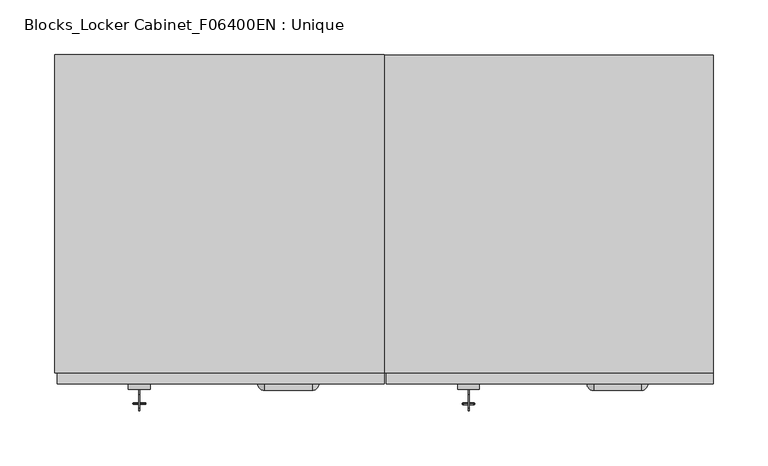
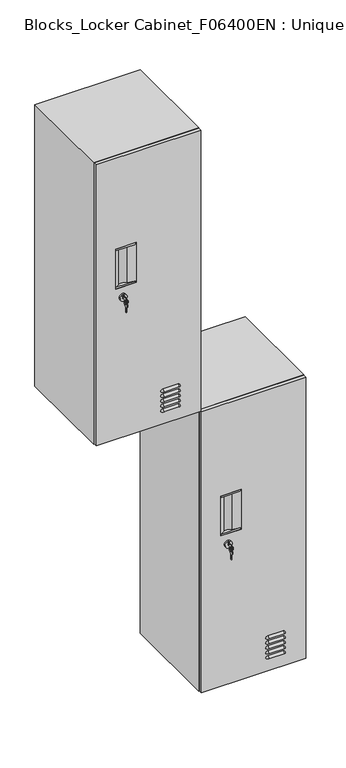
"""IFC4 building model written with IfcOpenShell, lengths in millimetres: furniture geometry, Blocks_Locker Cabinet_F06400EN : Unique."""

from ifc_helpers import new_model, si_unit, point, frame, frame_2d, origin, place, context, project, spatial, polyline, circle_curve, ellipse_curve, trimmed, segment, composite_curve, outline, extrude, faceted_brep, source, transform, mapped, element, save
from ifc_brep_helpers import plane_surface, cylinder_surface, revolved_surface, advanced_brep


def blocks_locker_cabinet_f06400en_unique_78fff643(model_context):
    return source(origin(), model_context, "Body", "SolidModel", [
        advanced_brep(
        [(-383.0, -12.5, 1375.0), (-363.0, -12.5, 1375.0), (-371.1588195, -12.5, 1382.0962926), (-371.1588195, -12.5, 1372.8618188), (-374.8411805, -12.5, 1372.8618188), (-374.8411805, -12.5, 1382.0962926), (-383.0, -7.5, 1375.0), (-363.0, -7.5, 1375.0), (-383.0, -10.7450625, 1375.0), (-363.0, -10.7450625, 1375.0), (-371.1588195, -10.7450625, 1382.0962926), (-371.1588195, -10.7450625, 1372.8618188), (-374.8411805, -10.7450625, 1372.8618188), (-374.8411805, -10.7450625, 1382.0962926)],
        [
            (0, 1, circle_curve(frame((-373.0, -12.5, 1375.0), z_axis=(0.0, -1.0, 0.0), x_axis=(1.0, 0.0, 0.0)), 10.0)),
            (1, 0, circle_curve(frame((-373.0, -12.5, 1375.0), z_axis=(0.0, -1.0, 0.0), x_axis=(1.0, 0.0, 0.0)), 10.0)),
            (2, 3),
            (3, 4),
            (4, 5),
            (5, 2),
            (6, 7, circle_curve(frame((-373.0, -7.5, 1375.0), z_axis=(0.0, 1.0, 0.0), x_axis=(1.0, 0.0, 0.0)), 10.0)),
            (7, 6, circle_curve(frame((-373.0, -7.5, 1375.0), z_axis=(0.0, 1.0, 0.0), x_axis=(1.0, 0.0, 0.0)), 10.0)),
            (0, 8),
            (8, 6),
            (7, 9),
            (9, 1),
            (2, 10),
            (10, 11),
            (11, 3),
            (11, 12),
            (12, 4),
            (12, 13),
            (13, 5),
            (13, 10),
        ],
        [
            plane_surface(frame((-363.0, -12.5, 1375.0), z_axis=(0.0, -1.0, 0.0), x_axis=(0.0, 0.0, 1.0))),
            plane_surface(frame((-363.0, -7.5, 1375.0), z_axis=(0.0, 1.0, 0.0), x_axis=(0.0, 0.0, -1.0))),
            cylinder_surface(frame((-373.0, -7.5, 1375.0), z_axis=(0.0, -1.0, 0.0), x_axis=(1.0, 0.0, 0.0)), 10.0),
            plane_surface(frame((-371.1588195, -12.5, 1382.0962926), z_axis=(-1.0, 0.0, 0.0), x_axis=(0.0, 1.0, 0.0))),
            plane_surface(frame((-371.1588195, -12.5, 1372.8618188), z_axis=(0.0, 0.0, 1.0), x_axis=(0.0, 1.0, 0.0))),
            plane_surface(frame((-374.8411805, -12.5, 1372.8618188), z_axis=(1.0, 0.0, 0.0), x_axis=(0.0, 1.0, 0.0))),
            plane_surface(frame((-374.8411805, -12.5, 1382.0962926), z_axis=(0.0, 0.0, -1.0), x_axis=(0.0, 1.0, 0.0))),
            plane_surface(frame((-363.0, -10.7450625, 1375.0), z_axis=(0.0, -1.0, 0.0), x_axis=(0.0, 0.0, 1.0))),
        ],
        [
            (0, [[1, 2], [3, 4, 5, 6]]),
            (1, [[7, 8]]),
            (2, [[-1, 9, 10, -8, 11, 12]]),
            (2, [[-2, -12, -11, -7, -10, -9]]),
            (3, [[-3, 13, 14, 15]]),
            (4, [[-4, -15, 16, 17]]),
            (5, [[-5, -17, 18, 19]]),
            (6, [[-6, -19, 20, -13]]),
            (7, [[-14, -20, -18, -16]]),
        ],
    ),
        extrude(outline(composite_curve([segment(trimmed(circle_curve(frame_2d((-23.0067332, 1375.0)), 6.5414185), [point((-16.8246351, 1372.8618188))], [point((-17.0336838, 1377.6669902))], False, "CARTESIAN"), True, "CONTINUOUS"), segment(polyline([(-17.0336838, 1377.6669902), (-10.7450625, 1377.6669902), (-10.7450625, 1372.8618188), (-12.0321832, 1372.8618188)]), True, "CONTINUOUS"), segment(trimmed(circle_curve(frame_2d((-12.908516, 1372.8618188)), 0.8763328), [point((-12.0321832, 1372.8618188))], [point((-13.7848488, 1372.8618188))], True, "CARTESIAN"), True, "CONTINUOUS"), segment(polyline([(-13.7848488, 1372.8618188), (-16.8246351, 1372.8618188)]), True, "CONTINUOUS")], self_intersect=False), holes=[composite_curve([segment(trimmed(circle_curve(frame_2d((-25.6281997, 1375.0)), 1.688217), [point((-27.3164167, 1375.0))], [point((-23.9399827, 1375.0))], True, "CARTESIAN"), True, "CONTINUOUS"), segment(trimmed(circle_curve(frame_2d((-25.6281997, 1375.0)), 1.688217), [point((-23.9399827, 1375.0))], [point((-27.3164167, 1375.0))], True, "CARTESIAN"), True, "CONTINUOUS")], self_intersect=False)]), frame((-373.4043078, 0.0, 0.0), z_axis=(1.0, 0.0, 0.0), x_axis=(0.0, 1.0, 0.0)), (0.0, 0.0, 1.0), 0.9157402),
        extrude(outline(composite_curve([segment(trimmed(circle_curve(frame_2d((-25.6743188, 1360.9839856)), 6.5414185), [point((-27.8125, 1354.8018875))], [point((-24.2573286, 1354.5978839))], False, "CARTESIAN"), True, "CONTINUOUS"), segment(polyline([(-24.2573286, 1354.5978839), (-24.2573286, 1337.7095301), (-25.9613419, 1337.7095301), (-27.8125, 1340.3532579), (-27.8125, 1342.0094356)]), True, "CONTINUOUS"), segment(trimmed(circle_curve(frame_2d((-27.8125, 1342.8857684)), 0.8763328), [point((-27.8125, 1342.0094356))], [point((-27.8125, 1343.7621012))], True, "CARTESIAN"), True, "CONTINUOUS"), segment(polyline([(-27.8125, 1343.7621012), (-27.8125, 1346.0094356)]), True, "CONTINUOUS"), segment(trimmed(circle_curve(frame_2d((-27.8125, 1346.8857684)), 0.8763328), [point((-27.8125, 1346.0094356))], [point((-27.8125, 1347.7621012))], True, "CARTESIAN"), True, "CONTINUOUS"), segment(polyline([(-27.8125, 1347.7621012), (-27.8125, 1350.0094356)]), True, "CONTINUOUS"), segment(trimmed(circle_curve(frame_2d((-27.8125, 1350.8857684)), 0.8763328), [point((-27.8125, 1350.0094356))], [point((-27.8125, 1351.7621012))], True, "CARTESIAN"), True, "CONTINUOUS"), segment(polyline([(-27.8125, 1351.7621012), (-27.8125, 1354.8018875)]), True, "CONTINUOUS")], self_intersect=False), holes=[composite_curve([segment(trimmed(circle_curve(frame_2d((-25.6743188, 1363.6054521)), 1.688217), [point((-25.6743188, 1365.2936691))], [point((-25.6743188, 1361.9172351))], True, "CARTESIAN"), True, "CONTINUOUS"), segment(trimmed(circle_curve(frame_2d((-25.6743188, 1363.6054521)), 1.688217), [point((-25.6743188, 1361.9172351))], [point((-25.6743188, 1365.2936691))], True, "CARTESIAN"), True, "CONTINUOUS")], self_intersect=False)]), frame((-373.4043078, 0.0, 0.0), z_axis=(1.0, 0.0, 0.0), x_axis=(0.0, 1.0, 0.0)), (0.0, 0.0, 1.0), 0.9157402),
        advanced_brep(
        [(-368.8, -25.663019, 1369.4000012), (-377.2, -25.663019, 1369.4000012), (-378.8, -25.663019, 1369.4000012), (-367.2, -25.663019, 1369.4000012)],
        [
            (0, 1, circle_curve(frame((-373.0, -25.663019, 1369.4000012), z_axis=(0.0, 1.0, 0.0), x_axis=(-1.0, 0.0, 0.0)), 4.2)),
            (1, 2, circle_curve(frame((-378.0, -25.663019, 1369.4000012), z_axis=(0.0, 0.0, -1.0), x_axis=(1.0, 0.0, 0.0)), 0.8)),
            (2, 3, circle_curve(frame((-373.0, -25.663019, 1369.4000012), z_axis=(0.0, -1.0, 0.0), x_axis=(-1.0, 0.0, 0.0)), 5.8)),
            (3, 0, circle_curve(frame((-368.0, -25.663019, 1369.4000012), z_axis=(0.0, 0.0, -1.0), x_axis=(-1.0, 0.0, 0.0)), 0.8)),
            (2, 1, circle_curve(frame((-378.0, -25.663019, 1369.4000012), z_axis=(0.0, 0.0, -1.0), x_axis=(1.0, 0.0, 0.0)), 0.8)),
            (0, 3, circle_curve(frame((-368.0, -25.663019, 1369.4000012), z_axis=(0.0, 0.0, -1.0), x_axis=(-1.0, 0.0, 0.0)), 0.8)),
            (1, 0, circle_curve(frame((-373.0, -25.663019, 1369.4000012), z_axis=(0.0, 1.0, 0.0), x_axis=(1.0, 0.0, 0.0)), 4.2)),
            (3, 2, circle_curve(frame((-373.0, -25.663019, 1369.4000012), z_axis=(0.0, -1.0, 0.0), x_axis=(1.0, 0.0, 0.0)), 5.8)),
        ],
        [
            revolved_surface(trimmed(ellipse_curve(frame((-378.0, -25.663019, 1369.4000012), z_axis=(0.0, 0.0, 1.0), x_axis=(1.0, 0.0, 0.0)), 0.8, 0.8), [point((-378.8, -25.663019, 1369.4000012))], [point((-377.2, -25.663019, 1369.4000012))], True, "CARTESIAN"), (-373.0, 2.5, 1369.4000012), (0.0, -1.0, 0.0)),
            revolved_surface(trimmed(ellipse_curve(frame((-378.0, -25.663019, 1369.4000012), z_axis=(0.0, 0.0, 1.0), x_axis=(1.0, 0.0, 0.0)), 0.8, 0.8), [point((-377.2, -25.663019, 1369.4000012))], [point((-378.8, -25.663019, 1369.4000012))], True, "CARTESIAN"), (-373.0, 2.5, 1369.4000012), (0.0, -1.0, 0.0)),
            revolved_surface(trimmed(ellipse_curve(frame((-368.0, -25.663019, 1369.4000012), z_axis=(0.0, 0.0, -1.0), x_axis=(-1.0, 0.0, 0.0)), 0.8, 0.8), [point((-367.2, -25.663019, 1369.4000012))], [point((-368.8, -25.663019, 1369.4000012))], True, "CARTESIAN"), (-373.0, 2.5, 1369.4000012), (0.0, -1.0, 0.0)),
            revolved_surface(trimmed(ellipse_curve(frame((-368.0, -25.663019, 1369.4000012), z_axis=(0.0, 0.0, -1.0), x_axis=(-1.0, 0.0, 0.0)), 0.8, 0.8), [point((-368.8, -25.663019, 1369.4000012))], [point((-367.2, -25.663019, 1369.4000012))], True, "CARTESIAN"), (-373.0, 2.5, 1369.4000012), (0.0, -1.0, 0.0)),
        ],
        [
            (0, [[1, 2, 3, 4]]),
            (1, [[-3, 5, -1, 6]]),
            (2, [[7, -4, 8, -2]]),
            (3, [[-8, -6, -7, -5]]),
        ],
    ),
        advanced_brep(
        [(-448.0, -7.5, 1799.0), (-150.0, -7.5, 1799.0), (-150.0, 2.5, 1799.0), (-448.0, 2.5, 1799.0), (-448.0, -7.5, 951.0), (-448.0, 2.5, 951.0), (-150.0, 2.5, 951.0), (-150.0, -7.5, 951.0), (-393.0, -7.5, 1525.0), (-333.7890736, -7.5, 1525.0), (-333.7890736, -7.5, 1405.0), (-393.0, -7.5, 1405.0), (-380.6526901, -0.3712773, 1525.0), (-357.2105549, -3.975278, 1525.0), (-380.6526901, -0.3712773, 1405.0), (-357.2105549, -3.975278, 1405.0)],
        [
            (0, 1),
            (1, 2),
            (2, 3),
            (3, 0),
            (4, 5),
            (5, 6),
            (6, 7),
            (7, 4),
            (0, 4),
            (7, 1),
            (8, 9),
            (9, 10),
            (10, 11),
            (11, 8),
            (6, 2),
            (5, 3),
            (12, 13, circle_curve(frame((-371.1776523, -16.7825242, 1525.0), z_axis=(0.0, 0.0, -1.0), x_axis=(0.0, -1.0, 0.0)), 18.9500756)),
            (13, 9),
            (8, 12),
            (14, 11),
            (10, 15),
            (15, 14, circle_curve(frame((-371.1776523, -16.7825242, 1405.0), z_axis=(0.0, 0.0, 1.0), x_axis=(0.0, -1.0, 0.0)), 18.9500756)),
            (14, 12),
            (13, 15),
        ],
        [
            plane_surface(frame((-150.0, -7.5, 1799.0), z_axis=(0.0, 0.0, 1.0), x_axis=(1.0, 0.0, 0.0))),
            plane_surface(frame((-150.0, -7.5, 951.0), z_axis=(0.0, 0.0, -1.0), x_axis=(-1.0, 0.0, 0.0))),
            plane_surface(frame((-448.0, -7.5, 1799.0), z_axis=(0.0, -1.0, 0.0), x_axis=(0.0, 0.0, -1.0))),
            plane_surface(frame((-150.0, -7.5, 1799.0), z_axis=(1.0, 0.0, 0.0), x_axis=(0.0, 0.0, -1.0))),
            plane_surface(frame((-150.0, 2.5, 1799.0), z_axis=(0.0, 1.0, 0.0), x_axis=(0.0, 0.0, -1.0))),
            plane_surface(frame((-448.0, 2.5, 1799.0), z_axis=(-1.0, 0.0, 0.0), x_axis=(0.0, 0.0, -1.0))),
            plane_surface(frame((-393.0, -7.5, 1525.0), z_axis=(0.0, 0.0, -1.0), x_axis=(-0.866025403784437, -0.5000000000000028, 0.0))),
            plane_surface(frame((-393.0, -7.5, 1405.0), z_axis=(0.0, 0.0, 1.0), x_axis=(0.866025403784437, 0.5000000000000028, 0.0))),
            plane_surface(frame((-380.6526901, -0.3712773, 1525.0), z_axis=(0.5000000000000028, -0.866025403784437, 0.0), x_axis=(0.0, 0.0, -1.0))),
            plane_surface(frame((-333.7890736, -7.5, 1525.0), z_axis=(-0.14881527984319862, -0.9888650122666847, 0.0), x_axis=(0.0, 0.0, -1.0))),
            revolved_surface(polyline([(-371.1776523, -35.7325998, 1525.0), (-371.1776523, -35.7325998, 1405.0)]), (-371.1776523, -16.7825242, 1405.0), (0.0, 0.0, 1.0)),
        ],
        [
            (0, [[1, 2, 3, 4]]),
            (1, [[5, 6, 7, 8]]),
            (2, [[-1, 9, -8, 10], [11, 12, 13, 14]]),
            (3, [[-2, -10, -7, 15]]),
            (4, [[-3, -15, -6, 16]]),
            (5, [[-4, -16, -5, -9]]),
            (6, [[17, 18, -11, 19]]),
            (7, [[20, -13, 21, 22]]),
            (8, [[-19, -14, -20, 23]]),
            (9, [[-18, 24, -21, -12]]),
            (10, [[-17, -23, -22, -24]]),
        ],
    ),
        advanced_brep(
        [(-265.0, -7.5, 991.0), (-259.0, -7.5, 997.0), (-215.4810333, -7.5, 997.0), (-209.4810333, -7.5, 991.0), (-215.4810333, -13.5, 991.0), (-259.0, -13.5, 991.0)],
        [
            (0, 1, circle_curve(frame((-259.0, -7.5, 991.0), z_axis=(0.0, 1.0, 0.0), x_axis=(1.0, 0.0, 0.0)), 6.0)),
            (1, 2),
            (2, 3, circle_curve(frame((-215.4810333, -7.5, 991.0), z_axis=(0.0, 1.0, 0.0), x_axis=(1.0, 0.0, 0.0)), 6.0)),
            (3, 0),
            (3, 4, circle_curve(frame((-215.4810333, -7.5, 991.0), z_axis=(0.0, 0.0, -1.0), x_axis=(1.0, 0.0, 0.0)), 6.0)),
            (4, 5),
            (5, 0, circle_curve(frame((-259.0, -7.5, 991.0), z_axis=(0.0, 0.0, -1.0), x_axis=(1.0, 0.0, 0.0)), 6.0)),
            (5, 1, circle_curve(frame((-259.0, -7.5, 991.0), z_axis=(-1.0, 0.0, 0.0), x_axis=(0.0, 0.0, 1.0)), 6.0)),
            (4, 2, circle_curve(frame((-215.4810333, -7.5, 991.0), z_axis=(-1.0, 0.0, 0.0), x_axis=(0.0, 0.0, 1.0)), 6.0)),
        ],
        [
            plane_surface(frame((-215.0, -7.5, 991.0), z_axis=(0.0, 1.0, 0.0), x_axis=(0.0, 0.0, 1.0))),
            plane_surface(frame((-215.0, -7.5, 991.0), z_axis=(0.0, 0.0, -1.0), x_axis=(0.0, -1.0, 0.0))),
            revolved_surface(trimmed(ellipse_curve(frame((-259.0, -7.5, 991.0), z_axis=(0.0, 1.0, 0.0), x_axis=(1.0, 0.0, 0.0)), 6.0, 6.0), [point((-265.0, -7.5, 991.0))], [point((-259.0, -7.5, 997.0))], True, "CARTESIAN"), (-215.0, -7.5, 991.0), (1.0, 0.0, 0.0)),
            cylinder_surface(frame((-215.0, -7.5, 991.0), z_axis=(1.0, 0.0, 0.0), x_axis=(0.0, 0.0, 1.0)), 6.0),
            revolved_surface(trimmed(ellipse_curve(frame((-215.4810333, -7.5, 991.0), z_axis=(0.0, 1.0, 0.0), x_axis=(1.0, 0.0, 0.0)), 6.0, 6.0), [point((-215.4810333, -7.5, 997.0))], [point((-209.4810333, -7.5, 991.0))], True, "CARTESIAN"), (-215.0, -7.5, 991.0), (1.0, 0.0, 0.0)),
        ],
        [
            (0, [[1, 2, 3, 4]]),
            (1, [[5, 6, 7, -4]]),
            (2, [[8, -1, -7]]),
            (3, [[9, -2, -8, -6]]),
            (4, [[-3, -9, -5]]),
        ],
    ),
        advanced_brep(
        [(-265.0, -7.5, 1006.0), (-259.0, -7.5, 1012.0), (-215.4810333, -7.5, 1012.0), (-209.4810333, -7.5, 1006.0), (-215.4810333, -13.5, 1006.0), (-259.0, -13.5, 1006.0)],
        [
            (0, 1, circle_curve(frame((-259.0, -7.5, 1006.0), z_axis=(0.0, 1.0, 0.0), x_axis=(1.0, 0.0, 0.0)), 6.0)),
            (1, 2),
            (2, 3, circle_curve(frame((-215.4810333, -7.5, 1006.0), z_axis=(0.0, 1.0, 0.0), x_axis=(1.0, 0.0, 0.0)), 6.0)),
            (3, 0),
            (3, 4, circle_curve(frame((-215.4810333, -7.5, 1006.0), z_axis=(0.0, 0.0, -1.0), x_axis=(1.0, 0.0, 0.0)), 6.0)),
            (4, 5),
            (5, 0, circle_curve(frame((-259.0, -7.5, 1006.0), z_axis=(0.0, 0.0, -1.0), x_axis=(1.0, 0.0, 0.0)), 6.0)),
            (5, 1, circle_curve(frame((-259.0, -7.5, 1006.0), z_axis=(-1.0, 0.0, 0.0), x_axis=(0.0, 0.0, 1.0)), 6.0)),
            (4, 2, circle_curve(frame((-215.4810333, -7.5, 1006.0), z_axis=(-1.0, 0.0, 0.0), x_axis=(0.0, 0.0, 1.0)), 6.0)),
        ],
        [
            plane_surface(frame((-215.0, -7.5, 1006.0), z_axis=(0.0, 1.0, 0.0), x_axis=(0.0, 0.0, 1.0))),
            plane_surface(frame((-215.0, -7.5, 1006.0), z_axis=(0.0, 0.0, -1.0), x_axis=(0.0, -1.0, 0.0))),
            revolved_surface(trimmed(ellipse_curve(frame((-259.0, -7.5, 1006.0), z_axis=(0.0, 1.0, 0.0), x_axis=(1.0, 0.0, 0.0)), 6.0, 6.0), [point((-265.0, -7.5, 1006.0))], [point((-259.0, -7.5, 1012.0))], True, "CARTESIAN"), (-215.0, -7.5, 1006.0), (1.0, 0.0, 0.0)),
            cylinder_surface(frame((-215.0, -7.5, 1006.0), z_axis=(1.0, 0.0, 0.0), x_axis=(0.0, 0.0, 1.0)), 6.0),
            revolved_surface(trimmed(ellipse_curve(frame((-215.4810333, -7.5, 1006.0), z_axis=(0.0, 1.0, 0.0), x_axis=(1.0, 0.0, 0.0)), 6.0, 6.0), [point((-215.4810333, -7.5, 1012.0))], [point((-209.4810333, -7.5, 1006.0))], True, "CARTESIAN"), (-215.0, -7.5, 1006.0), (1.0, 0.0, 0.0)),
        ],
        [
            (0, [[1, 2, 3, 4]]),
            (1, [[5, 6, 7, -4]]),
            (2, [[8, -1, -7]]),
            (3, [[9, -2, -8, -6]]),
            (4, [[-3, -9, -5]]),
        ],
    ),
        advanced_brep(
        [(-265.0, -7.5, 1021.0), (-259.0, -7.5, 1027.0), (-215.4810333, -7.5, 1027.0), (-209.4810333, -7.5, 1021.0), (-215.4810333, -13.5, 1021.0), (-259.0, -13.5, 1021.0)],
        [
            (0, 1, circle_curve(frame((-259.0, -7.5, 1021.0), z_axis=(0.0, 1.0, 0.0), x_axis=(1.0, 0.0, 0.0)), 6.0)),
            (1, 2),
            (2, 3, circle_curve(frame((-215.4810333, -7.5, 1021.0), z_axis=(0.0, 1.0, 0.0), x_axis=(1.0, 0.0, 0.0)), 6.0)),
            (3, 0),
            (3, 4, circle_curve(frame((-215.4810333, -7.5, 1021.0), z_axis=(0.0, 0.0, -1.0), x_axis=(1.0, 0.0, 0.0)), 6.0)),
            (4, 5),
            (5, 0, circle_curve(frame((-259.0, -7.5, 1021.0), z_axis=(0.0, 0.0, -1.0), x_axis=(1.0, 0.0, 0.0)), 6.0)),
            (5, 1, circle_curve(frame((-259.0, -7.5, 1021.0), z_axis=(-1.0, 0.0, 0.0), x_axis=(0.0, 0.0, 1.0)), 6.0)),
            (4, 2, circle_curve(frame((-215.4810333, -7.5, 1021.0), z_axis=(-1.0, 0.0, 0.0), x_axis=(0.0, 0.0, 1.0)), 6.0)),
        ],
        [
            plane_surface(frame((-215.0, -7.5, 1021.0), z_axis=(0.0, 1.0, 0.0), x_axis=(0.0, 0.0, 1.0))),
            plane_surface(frame((-215.0, -7.5, 1021.0), z_axis=(0.0, 0.0, -1.0), x_axis=(0.0, -1.0, 0.0))),
            revolved_surface(trimmed(ellipse_curve(frame((-259.0, -7.5, 1021.0), z_axis=(0.0, 1.0, 0.0), x_axis=(1.0, 0.0, 0.0)), 6.0, 6.0), [point((-265.0, -7.5, 1021.0))], [point((-259.0, -7.5, 1027.0))], True, "CARTESIAN"), (-215.0, -7.5, 1021.0), (1.0, 0.0, 0.0)),
            cylinder_surface(frame((-215.0, -7.5, 1021.0), z_axis=(1.0, 0.0, 0.0), x_axis=(0.0, 0.0, 1.0)), 6.0),
            revolved_surface(trimmed(ellipse_curve(frame((-215.4810333, -7.5, 1021.0), z_axis=(0.0, 1.0, 0.0), x_axis=(1.0, 0.0, 0.0)), 6.0, 6.0), [point((-215.4810333, -7.5, 1027.0))], [point((-209.4810333, -7.5, 1021.0))], True, "CARTESIAN"), (-215.0, -7.5, 1021.0), (1.0, 0.0, 0.0)),
        ],
        [
            (0, [[1, 2, 3, 4]]),
            (1, [[5, 6, 7, -4]]),
            (2, [[8, -1, -7]]),
            (3, [[9, -2, -8, -6]]),
            (4, [[-3, -9, -5]]),
        ],
    ),
        advanced_brep(
        [(-265.0, -7.5, 1036.0), (-259.0, -7.5, 1042.0), (-215.4810333, -7.5, 1042.0), (-209.4810333, -7.5, 1036.0), (-215.4810333, -13.5, 1036.0), (-259.0, -13.5, 1036.0)],
        [
            (0, 1, circle_curve(frame((-259.0, -7.5, 1036.0), z_axis=(0.0, 1.0, 0.0), x_axis=(1.0, 0.0, 0.0)), 6.0)),
            (1, 2),
            (2, 3, circle_curve(frame((-215.4810333, -7.5, 1036.0), z_axis=(0.0, 1.0, 0.0), x_axis=(1.0, 0.0, 0.0)), 6.0)),
            (3, 0),
            (3, 4, circle_curve(frame((-215.4810333, -7.5, 1036.0), z_axis=(0.0, 0.0, -1.0), x_axis=(1.0, 0.0, 0.0)), 6.0)),
            (4, 5),
            (5, 0, circle_curve(frame((-259.0, -7.5, 1036.0), z_axis=(0.0, 0.0, -1.0), x_axis=(1.0, 0.0, 0.0)), 6.0)),
            (5, 1, circle_curve(frame((-259.0, -7.5, 1036.0), z_axis=(-1.0, 0.0, 0.0), x_axis=(0.0, 0.0, 1.0)), 6.0)),
            (4, 2, circle_curve(frame((-215.4810333, -7.5, 1036.0), z_axis=(-1.0, 0.0, 0.0), x_axis=(0.0, 0.0, 1.0)), 6.0)),
        ],
        [
            plane_surface(frame((-215.0, -7.5, 1036.0), z_axis=(0.0, 1.0, 0.0), x_axis=(0.0, 0.0, 1.0))),
            plane_surface(frame((-215.0, -7.5, 1036.0), z_axis=(0.0, 0.0, -1.0), x_axis=(0.0, -1.0, 0.0))),
            revolved_surface(trimmed(ellipse_curve(frame((-259.0, -7.5, 1036.0), z_axis=(0.0, 1.0, 0.0), x_axis=(1.0, 0.0, 0.0)), 6.0, 6.0), [point((-265.0, -7.5, 1036.0))], [point((-259.0, -7.5, 1042.0))], True, "CARTESIAN"), (-215.0, -7.5, 1036.0), (1.0, 0.0, 0.0)),
            cylinder_surface(frame((-215.0, -7.5, 1036.0), z_axis=(1.0, 0.0, 0.0), x_axis=(0.0, 0.0, 1.0)), 6.0),
            revolved_surface(trimmed(ellipse_curve(frame((-215.4810333, -7.5, 1036.0), z_axis=(0.0, 1.0, 0.0), x_axis=(1.0, 0.0, 0.0)), 6.0, 6.0), [point((-215.4810333, -7.5, 1042.0))], [point((-209.4810333, -7.5, 1036.0))], True, "CARTESIAN"), (-215.0, -7.5, 1036.0), (1.0, 0.0, 0.0)),
        ],
        [
            (0, [[1, 2, 3, 4]]),
            (1, [[5, 6, 7, -4]]),
            (2, [[8, -1, -7]]),
            (3, [[9, -2, -8, -6]]),
            (4, [[-3, -9, -5]]),
        ],
    ),
        advanced_brep(
        [(-265.0, -7.5, 1051.0), (-259.0, -7.5, 1057.0), (-215.4810333, -7.5, 1057.0), (-209.4810333, -7.5, 1051.0), (-215.4810333, -13.5, 1051.0), (-259.0, -13.5, 1051.0)],
        [
            (0, 1, circle_curve(frame((-259.0, -7.5, 1051.0), z_axis=(0.0, 1.0, 0.0), x_axis=(1.0, 0.0, 0.0)), 6.0)),
            (1, 2),
            (2, 3, circle_curve(frame((-215.4810333, -7.5, 1051.0), z_axis=(0.0, 1.0, 0.0), x_axis=(1.0, 0.0, 0.0)), 6.0)),
            (3, 0),
            (3, 4, circle_curve(frame((-215.4810333, -7.5, 1051.0), z_axis=(0.0, 0.0, -1.0), x_axis=(1.0, 0.0, 0.0)), 6.0)),
            (4, 5),
            (5, 0, circle_curve(frame((-259.0, -7.5, 1051.0), z_axis=(0.0, 0.0, -1.0), x_axis=(1.0, 0.0, 0.0)), 6.0)),
            (5, 1, circle_curve(frame((-259.0, -7.5, 1051.0), z_axis=(-1.0, 0.0, 0.0), x_axis=(0.0, 0.0, 1.0)), 6.0)),
            (4, 2, circle_curve(frame((-215.4810333, -7.5, 1051.0), z_axis=(-1.0, 0.0, 0.0), x_axis=(0.0, 0.0, 1.0)), 6.0)),
        ],
        [
            plane_surface(frame((-215.0, -7.5, 1051.0), z_axis=(0.0, 1.0, 0.0), x_axis=(0.0, 0.0, 1.0))),
            plane_surface(frame((-215.0, -7.5, 1051.0), z_axis=(0.0, 0.0, -1.0), x_axis=(0.0, -1.0, 0.0))),
            revolved_surface(trimmed(ellipse_curve(frame((-259.0, -7.5, 1051.0), z_axis=(0.0, 1.0, 0.0), x_axis=(1.0, 0.0, 0.0)), 6.0, 6.0), [point((-265.0, -7.5, 1051.0))], [point((-259.0, -7.5, 1057.0))], True, "CARTESIAN"), (-215.0, -7.5, 1051.0), (1.0, 0.0, 0.0)),
            cylinder_surface(frame((-215.0, -7.5, 1051.0), z_axis=(1.0, 0.0, 0.0), x_axis=(0.0, 0.0, 1.0)), 6.0),
            revolved_surface(trimmed(ellipse_curve(frame((-215.4810333, -7.5, 1051.0), z_axis=(0.0, 1.0, 0.0), x_axis=(1.0, 0.0, 0.0)), 6.0, 6.0), [point((-215.4810333, -7.5, 1057.0))], [point((-209.4810333, -7.5, 1051.0))], True, "CARTESIAN"), (-215.0, -7.5, 1051.0), (1.0, 0.0, 0.0)),
        ],
        [
            (0, [[1, 2, 3, 4]]),
            (1, [[5, 6, 7, -4]]),
            (2, [[8, -1, -7]]),
            (3, [[9, -2, -8, -6]]),
            (4, [[-3, -9, -5]]),
        ],
    ),
        extrude(outline(composite_curve([segment(trimmed(circle_curve(frame_2d((-371.1776523, -16.7825242)), 18.9500756), [point((-380.6526901, -0.3712773))], [point((-357.2105549, -3.975278))], False, "CARTESIAN"), True, "CONTINUOUS"), segment(polyline([(-357.2105549, -3.975278), (-333.7890736, -7.5), (-393.0, -7.5), (-380.6526901, -0.3712773)]), True, "CONTINUOUS")], self_intersect=False)), frame((0.0, 0.0, 1405.0), z_axis=(0.0, 0.0, 1.0), x_axis=(1.0, 0.0, 0.0)), (0.0, 0.0, 1.0), 5.0),
        extrude(outline(composite_curve([segment(trimmed(circle_curve(frame_2d((-371.1776523, -16.7825242)), 18.9500756), [point((-380.6526901, -0.3712773))], [point((-357.2105549, -3.975278))], False, "CARTESIAN"), True, "CONTINUOUS"), segment(polyline([(-357.2105549, -3.975278), (-333.7890736, -7.5), (-393.0, -7.5), (-380.6526901, -0.3712773)]), True, "CONTINUOUS")], self_intersect=False)), frame((0.0, 0.0, 1520.0), z_axis=(0.0, 0.0, 1.0), x_axis=(1.0, 0.0, 0.0)), (0.0, 0.0, 1.0), 5.0),
        faceted_brep([(-150.0, 2.5, 1800.0), (-450.0, 2.5, 1800.0), (-450.0, 2.5, 950.0), (-150.0, 2.5, 950.0), (-160.0, 2.5, 1790.0), (-160.0, 2.5, 960.0), (-440.0, 2.5, 960.0), (-440.0, 2.5, 1790.0), (-150.0, 292.5, 1800.0), (-150.0, 292.5, 950.0), (-450.0, 292.5, 950.0), (-450.0, 292.5, 1800.0), (-150.0, 282.5, 1800.0), (-450.0, 282.5, 1800.0), (-450.0, 282.5, 950.0), (-150.0, 282.5, 950.0), (-160.0, 282.5, 1790.0), (-160.0, 282.5, 960.0), (-440.0, 282.5, 960.0), (-440.0, 282.5, 1790.0)], [[[0, 1, 2, 3], [4, 5, 6, 7]], [[8, 9, 10, 11]], [[1, 0, 12, 8, 11, 13]], [[2, 1, 13, 11, 10, 14]], [[3, 2, 14, 10, 9, 15]], [[0, 3, 15, 9, 8, 12]], [[5, 4, 16, 17]], [[6, 5, 17, 18]], [[7, 6, 18, 19]], [[4, 7, 19, 16]], [[17, 16, 19, 18]]]),
        advanced_brep(
        [(-83.0, -12.5, 525.0), (-63.0, -12.5, 525.0), (-71.1588195, -12.5, 532.0962926), (-71.1588195, -12.5, 522.8618188), (-74.8411805, -12.5, 522.8618188), (-74.8411805, -12.5, 532.0962926), (-83.0, -7.5, 525.0), (-63.0, -7.5, 525.0), (-83.0, -10.7450625, 525.0), (-63.0, -10.7450625, 525.0), (-71.1588195, -10.7450625, 532.0962926), (-71.1588195, -10.7450625, 522.8618188), (-74.8411805, -10.7450625, 522.8618188), (-74.8411805, -10.7450625, 532.0962926)],
        [
            (0, 1, circle_curve(frame((-73.0, -12.5, 525.0), z_axis=(0.0, -1.0, 0.0), x_axis=(1.0, 0.0, 0.0)), 10.0)),
            (1, 0, circle_curve(frame((-73.0, -12.5, 525.0), z_axis=(0.0, -1.0, 0.0), x_axis=(1.0, 0.0, 0.0)), 10.0)),
            (2, 3),
            (3, 4),
            (4, 5),
            (5, 2),
            (6, 7, circle_curve(frame((-73.0, -7.5, 525.0), z_axis=(0.0, 1.0, 0.0), x_axis=(1.0, 0.0, 0.0)), 10.0)),
            (7, 6, circle_curve(frame((-73.0, -7.5, 525.0), z_axis=(0.0, 1.0, 0.0), x_axis=(1.0, 0.0, 0.0)), 10.0)),
            (0, 8),
            (8, 6),
            (7, 9),
            (9, 1),
            (2, 10),
            (10, 11),
            (11, 3),
            (11, 12),
            (12, 4),
            (12, 13),
            (13, 5),
            (13, 10),
        ],
        [
            plane_surface(frame((-63.0, -12.5, 525.0), z_axis=(0.0, -1.0, 0.0), x_axis=(0.0, 0.0, 1.0))),
            plane_surface(frame((-63.0, -7.5, 525.0), z_axis=(0.0, 1.0, 0.0), x_axis=(0.0, 0.0, -1.0))),
            cylinder_surface(frame((-73.0, -7.5, 525.0), z_axis=(0.0, -1.0, 0.0), x_axis=(1.0, 0.0, 0.0)), 10.0),
            plane_surface(frame((-71.1588195, -12.5, 532.0962926), z_axis=(-1.0, 0.0, 0.0), x_axis=(0.0, 1.0, 0.0))),
            plane_surface(frame((-71.1588195, -12.5, 522.8618188), z_axis=(0.0, 0.0, 1.0), x_axis=(0.0, 1.0, 0.0))),
            plane_surface(frame((-74.8411805, -12.5, 522.8618188), z_axis=(1.0, 0.0, 0.0), x_axis=(0.0, 1.0, 0.0))),
            plane_surface(frame((-74.8411805, -12.5, 532.0962926), z_axis=(0.0, 0.0, -1.0), x_axis=(0.0, 1.0, 0.0))),
            plane_surface(frame((-63.0, -10.7450625, 525.0), z_axis=(0.0, -1.0, 0.0), x_axis=(0.0, 0.0, 1.0))),
        ],
        [
            (0, [[1, 2], [3, 4, 5, 6]]),
            (1, [[7, 8]]),
            (2, [[-1, 9, 10, -8, 11, 12]]),
            (2, [[-2, -12, -11, -7, -10, -9]]),
            (3, [[-3, 13, 14, 15]]),
            (4, [[-4, -15, 16, 17]]),
            (5, [[-5, -17, 18, 19]]),
            (6, [[-6, -19, 20, -13]]),
            (7, [[-14, -20, -18, -16]]),
        ],
    ),
        extrude(outline(composite_curve([segment(trimmed(circle_curve(frame_2d((-23.0067332, 525.0)), 6.5414185), [point((-16.8246351, 522.8618188))], [point((-17.0336838, 527.6669902))], False, "CARTESIAN"), True, "CONTINUOUS"), segment(polyline([(-17.0336838, 527.6669902), (-10.7450625, 527.6669902), (-10.7450625, 522.8618188), (-12.0321832, 522.8618188)]), True, "CONTINUOUS"), segment(trimmed(circle_curve(frame_2d((-12.908516, 522.8618188)), 0.8763328), [point((-12.0321832, 522.8618188))], [point((-13.7848488, 522.8618188))], True, "CARTESIAN"), True, "CONTINUOUS"), segment(polyline([(-13.7848488, 522.8618188), (-16.8246351, 522.8618188)]), True, "CONTINUOUS")], self_intersect=False), holes=[composite_curve([segment(trimmed(circle_curve(frame_2d((-25.6281997, 525.0)), 1.688217), [point((-27.3164167, 525.0))], [point((-23.9399827, 525.0))], True, "CARTESIAN"), True, "CONTINUOUS"), segment(trimmed(circle_curve(frame_2d((-25.6281997, 525.0)), 1.688217), [point((-23.9399827, 525.0))], [point((-27.3164167, 525.0))], True, "CARTESIAN"), True, "CONTINUOUS")], self_intersect=False)]), frame((-73.4043078, 0.0, 0.0), z_axis=(1.0, 0.0, 0.0), x_axis=(0.0, 1.0, 0.0)), (0.0, 0.0, 1.0), 0.9157402),
        extrude(outline(composite_curve([segment(trimmed(circle_curve(frame_2d((-25.6743188, 510.9839856)), 6.5414185), [point((-27.8125, 504.8018875))], [point((-24.2573286, 504.5978839))], False, "CARTESIAN"), True, "CONTINUOUS"), segment(polyline([(-24.2573286, 504.5978839), (-24.2573286, 487.7095301), (-25.9613419, 487.7095301), (-27.8125, 490.3532579), (-27.8125, 492.0094356)]), True, "CONTINUOUS"), segment(trimmed(circle_curve(frame_2d((-27.8125, 492.8857684)), 0.8763328), [point((-27.8125, 492.0094356))], [point((-27.8125, 493.7621012))], True, "CARTESIAN"), True, "CONTINUOUS"), segment(polyline([(-27.8125, 493.7621012), (-27.8125, 496.0094356)]), True, "CONTINUOUS"), segment(trimmed(circle_curve(frame_2d((-27.8125, 496.8857684)), 0.8763328), [point((-27.8125, 496.0094356))], [point((-27.8125, 497.7621012))], True, "CARTESIAN"), True, "CONTINUOUS"), segment(polyline([(-27.8125, 497.7621012), (-27.8125, 500.0094356)]), True, "CONTINUOUS"), segment(trimmed(circle_curve(frame_2d((-27.8125, 500.8857684)), 0.8763328), [point((-27.8125, 500.0094356))], [point((-27.8125, 501.7621012))], True, "CARTESIAN"), True, "CONTINUOUS"), segment(polyline([(-27.8125, 501.7621012), (-27.8125, 504.8018875)]), True, "CONTINUOUS")], self_intersect=False), holes=[composite_curve([segment(trimmed(circle_curve(frame_2d((-25.6743188, 513.6054521)), 1.688217), [point((-25.6743188, 515.2936691))], [point((-25.6743188, 511.9172351))], True, "CARTESIAN"), True, "CONTINUOUS"), segment(trimmed(circle_curve(frame_2d((-25.6743188, 513.6054521)), 1.688217), [point((-25.6743188, 511.9172351))], [point((-25.6743188, 515.2936691))], True, "CARTESIAN"), True, "CONTINUOUS")], self_intersect=False)]), frame((-73.4043078, 0.0, 0.0), z_axis=(1.0, 0.0, 0.0), x_axis=(0.0, 1.0, 0.0)), (0.0, 0.0, 1.0), 0.9157402),
        advanced_brep(
        [(-68.8, -25.663019, 519.4000012), (-77.2, -25.663019, 519.4000012), (-78.8, -25.663019, 519.4000012), (-67.2, -25.663019, 519.4000012)],
        [
            (0, 1, circle_curve(frame((-73.0, -25.663019, 519.4000012), z_axis=(0.0, 1.0, 0.0), x_axis=(-1.0, 0.0, 0.0)), 4.2)),
            (1, 2, circle_curve(frame((-78.0, -25.663019, 519.4000012), z_axis=(0.0, 0.0, -1.0), x_axis=(1.0, 0.0, 0.0)), 0.8)),
            (2, 3, circle_curve(frame((-73.0, -25.663019, 519.4000012), z_axis=(0.0, -1.0, 0.0), x_axis=(-1.0, 0.0, 0.0)), 5.8)),
            (3, 0, circle_curve(frame((-68.0, -25.663019, 519.4000012), z_axis=(0.0, 0.0, -1.0), x_axis=(-1.0, 0.0, 0.0)), 0.8)),
            (2, 1, circle_curve(frame((-78.0, -25.663019, 519.4000012), z_axis=(0.0, 0.0, -1.0), x_axis=(1.0, 0.0, 0.0)), 0.8)),
            (0, 3, circle_curve(frame((-68.0, -25.663019, 519.4000012), z_axis=(0.0, 0.0, -1.0), x_axis=(-1.0, 0.0, 0.0)), 0.8)),
            (1, 0, circle_curve(frame((-73.0, -25.663019, 519.4000012), z_axis=(0.0, 1.0, 0.0), x_axis=(1.0, 0.0, 0.0)), 4.2)),
            (3, 2, circle_curve(frame((-73.0, -25.663019, 519.4000012), z_axis=(0.0, -1.0, 0.0), x_axis=(1.0, 0.0, 0.0)), 5.8)),
        ],
        [
            revolved_surface(trimmed(ellipse_curve(frame((-78.0, -25.663019, 519.4000012), z_axis=(0.0, 0.0, 1.0), x_axis=(1.0, 0.0, 0.0)), 0.8, 0.8), [point((-78.8, -25.663019, 519.4000012))], [point((-77.2, -25.663019, 519.4000012))], True, "CARTESIAN"), (-73.0, 2.5, 519.4000012), (0.0, -1.0, 0.0)),
            revolved_surface(trimmed(ellipse_curve(frame((-78.0, -25.663019, 519.4000012), z_axis=(0.0, 0.0, 1.0), x_axis=(1.0, 0.0, 0.0)), 0.8, 0.8), [point((-77.2, -25.663019, 519.4000012))], [point((-78.8, -25.663019, 519.4000012))], True, "CARTESIAN"), (-73.0, 2.5, 519.4000012), (0.0, -1.0, 0.0)),
            revolved_surface(trimmed(ellipse_curve(frame((-68.0, -25.663019, 519.4000012), z_axis=(0.0, 0.0, -1.0), x_axis=(-1.0, 0.0, 0.0)), 0.8, 0.8), [point((-67.2, -25.663019, 519.4000012))], [point((-68.8, -25.663019, 519.4000012))], True, "CARTESIAN"), (-73.0, 2.5, 519.4000012), (0.0, -1.0, 0.0)),
            revolved_surface(trimmed(ellipse_curve(frame((-68.0, -25.663019, 519.4000012), z_axis=(0.0, 0.0, -1.0), x_axis=(-1.0, 0.0, 0.0)), 0.8, 0.8), [point((-68.8, -25.663019, 519.4000012))], [point((-67.2, -25.663019, 519.4000012))], True, "CARTESIAN"), (-73.0, 2.5, 519.4000012), (0.0, -1.0, 0.0)),
        ],
        [
            (0, [[1, 2, 3, 4]]),
            (1, [[-3, 5, -1, 6]]),
            (2, [[7, -4, 8, -2]]),
            (3, [[-8, -6, -7, -5]]),
        ],
    ),
        advanced_brep(
        [(-148.0, -7.5, 949.0), (150.0, -7.5, 949.0), (150.0, 2.5, 949.0), (-148.0, 2.5, 949.0), (-148.0, -7.5, 101.0), (-148.0, 2.5, 101.0), (150.0, 2.5, 101.0), (150.0, -7.5, 101.0), (-93.0, -7.5, 675.0), (-33.7890736, -7.5, 675.0), (-33.7890736, -7.5, 555.0), (-93.0, -7.5, 555.0), (-80.6526901, -0.3712773, 675.0), (-57.2105549, -3.975278, 675.0), (-80.6526901, -0.3712773, 555.0), (-57.2105549, -3.975278, 555.0)],
        [
            (0, 1),
            (1, 2),
            (2, 3),
            (3, 0),
            (4, 5),
            (5, 6),
            (6, 7),
            (7, 4),
            (0, 4),
            (7, 1),
            (8, 9),
            (9, 10),
            (10, 11),
            (11, 8),
            (6, 2),
            (5, 3),
            (12, 13, circle_curve(frame((-71.1776523, -16.7825242, 675.0), z_axis=(0.0, 0.0, -1.0), x_axis=(0.0, -1.0, 0.0)), 18.9500756)),
            (13, 9),
            (8, 12),
            (14, 11),
            (10, 15),
            (15, 14, circle_curve(frame((-71.1776523, -16.7825242, 555.0), z_axis=(0.0, 0.0, 1.0), x_axis=(0.0, -1.0, 0.0)), 18.9500756)),
            (14, 12),
            (13, 15),
        ],
        [
            plane_surface(frame((150.0, -7.5, 949.0), z_axis=(0.0, 0.0, 1.0), x_axis=(1.0, 0.0, 0.0))),
            plane_surface(frame((150.0, -7.5, 101.0), z_axis=(0.0, 0.0, -1.0), x_axis=(-1.0, 0.0, 0.0))),
            plane_surface(frame((-148.0, -7.5, 949.0), z_axis=(0.0, -1.0, 0.0), x_axis=(0.0, 0.0, -1.0))),
            plane_surface(frame((150.0, -7.5, 949.0), z_axis=(1.0, 0.0, 0.0), x_axis=(0.0, 0.0, -1.0))),
            plane_surface(frame((150.0, 2.5, 949.0), z_axis=(0.0, 1.0, 0.0), x_axis=(0.0, 0.0, -1.0))),
            plane_surface(frame((-148.0, 2.5, 949.0), z_axis=(-1.0, 0.0, 0.0), x_axis=(0.0, 0.0, -1.0))),
            plane_surface(frame((-93.0, -7.5, 675.0), z_axis=(0.0, 0.0, -1.0), x_axis=(-0.866025403784437, -0.5000000000000028, 0.0))),
            plane_surface(frame((-93.0, -7.5, 555.0), z_axis=(0.0, 0.0, 1.0), x_axis=(0.866025403784437, 0.5000000000000028, 0.0))),
            plane_surface(frame((-80.6526901, -0.3712773, 675.0), z_axis=(0.5000000000000028, -0.866025403784437, 0.0), x_axis=(0.0, 0.0, -1.0))),
            plane_surface(frame((-33.7890736, -7.5, 675.0), z_axis=(-0.14881527984319862, -0.9888650122666847, 0.0), x_axis=(0.0, 0.0, -1.0))),
            revolved_surface(polyline([(-71.1776523, -35.7325998, 675.0), (-71.1776523, -35.7325998, 555.0)]), (-71.1776523, -16.7825242, 555.0), (0.0, 0.0, 1.0)),
        ],
        [
            (0, [[1, 2, 3, 4]]),
            (1, [[5, 6, 7, 8]]),
            (2, [[-1, 9, -8, 10], [11, 12, 13, 14]]),
            (3, [[-2, -10, -7, 15]]),
            (4, [[-3, -15, -6, 16]]),
            (5, [[-4, -16, -5, -9]]),
            (6, [[17, 18, -11, 19]]),
            (7, [[20, -13, 21, 22]]),
            (8, [[-19, -14, -20, 23]]),
            (9, [[-18, 24, -21, -12]]),
            (10, [[-17, -23, -22, -24]]),
        ],
    ),
        advanced_brep(
        [(35.0, -7.5, 141.0), (41.0, -7.5, 147.0), (84.5189667, -7.5, 147.0), (90.5189667, -7.5, 141.0), (84.5189667, -13.5, 141.0), (41.0, -13.5, 141.0)],
        [
            (0, 1, circle_curve(frame((41.0, -7.5, 141.0), z_axis=(0.0, 1.0, 0.0), x_axis=(1.0, 0.0, 0.0)), 6.0)),
            (1, 2),
            (2, 3, circle_curve(frame((84.5189667, -7.5, 141.0), z_axis=(0.0, 1.0, 0.0), x_axis=(1.0, 0.0, 0.0)), 6.0)),
            (3, 0),
            (3, 4, circle_curve(frame((84.5189667, -7.5, 141.0), z_axis=(0.0, 0.0, -1.0), x_axis=(1.0, 0.0, 0.0)), 6.0)),
            (4, 5),
            (5, 0, circle_curve(frame((41.0, -7.5, 141.0), z_axis=(0.0, 0.0, -1.0), x_axis=(1.0, 0.0, 0.0)), 6.0)),
            (5, 1, circle_curve(frame((41.0, -7.5, 141.0), z_axis=(-1.0, 0.0, 0.0), x_axis=(0.0, 0.0, 1.0)), 6.0)),
            (4, 2, circle_curve(frame((84.5189667, -7.5, 141.0), z_axis=(-1.0, 0.0, 0.0), x_axis=(0.0, 0.0, 1.0)), 6.0)),
        ],
        [
            plane_surface(frame((85.0, -7.5, 141.0), z_axis=(0.0, 1.0, 0.0), x_axis=(0.0, 0.0, 1.0))),
            plane_surface(frame((85.0, -7.5, 141.0), z_axis=(0.0, 0.0, -1.0), x_axis=(0.0, -1.0, 0.0))),
            revolved_surface(trimmed(ellipse_curve(frame((41.0, -7.5, 141.0), z_axis=(0.0, 1.0, 0.0), x_axis=(1.0, 0.0, 0.0)), 6.0, 6.0), [point((35.0, -7.5, 141.0))], [point((41.0, -7.5, 147.0))], True, "CARTESIAN"), (85.0, -7.5, 141.0), (1.0, 0.0, 0.0)),
            cylinder_surface(frame((85.0, -7.5, 141.0), z_axis=(1.0, 0.0, 0.0), x_axis=(0.0, 0.0, 1.0)), 6.0),
            revolved_surface(trimmed(ellipse_curve(frame((84.5189667, -7.5, 141.0), z_axis=(0.0, 1.0, 0.0), x_axis=(1.0, 0.0, 0.0)), 6.0, 6.0), [point((84.5189667, -7.5, 147.0))], [point((90.5189667, -7.5, 141.0))], True, "CARTESIAN"), (85.0, -7.5, 141.0), (1.0, 0.0, 0.0)),
        ],
        [
            (0, [[1, 2, 3, 4]]),
            (1, [[5, 6, 7, -4]]),
            (2, [[8, -1, -7]]),
            (3, [[9, -2, -8, -6]]),
            (4, [[-3, -9, -5]]),
        ],
    ),
        advanced_brep(
        [(35.0, -7.5, 156.0), (41.0, -7.5, 162.0), (84.5189667, -7.5, 162.0), (90.5189667, -7.5, 156.0), (84.5189667, -13.5, 156.0), (41.0, -13.5, 156.0)],
        [
            (0, 1, circle_curve(frame((41.0, -7.5, 156.0), z_axis=(0.0, 1.0, 0.0), x_axis=(1.0, 0.0, 0.0)), 6.0)),
            (1, 2),
            (2, 3, circle_curve(frame((84.5189667, -7.5, 156.0), z_axis=(0.0, 1.0, 0.0), x_axis=(1.0, 0.0, 0.0)), 6.0)),
            (3, 0),
            (3, 4, circle_curve(frame((84.5189667, -7.5, 156.0), z_axis=(0.0, 0.0, -1.0), x_axis=(1.0, 0.0, 0.0)), 6.0)),
            (4, 5),
            (5, 0, circle_curve(frame((41.0, -7.5, 156.0), z_axis=(0.0, 0.0, -1.0), x_axis=(1.0, 0.0, 0.0)), 6.0)),
            (5, 1, circle_curve(frame((41.0, -7.5, 156.0), z_axis=(-1.0, 0.0, 0.0), x_axis=(0.0, 0.0, 1.0)), 6.0)),
            (4, 2, circle_curve(frame((84.5189667, -7.5, 156.0), z_axis=(-1.0, 0.0, 0.0), x_axis=(0.0, 0.0, 1.0)), 6.0)),
        ],
        [
            plane_surface(frame((85.0, -7.5, 156.0), z_axis=(0.0, 1.0, 0.0), x_axis=(0.0, 0.0, 1.0))),
            plane_surface(frame((85.0, -7.5, 156.0), z_axis=(0.0, 0.0, -1.0), x_axis=(0.0, -1.0, 0.0))),
            revolved_surface(trimmed(ellipse_curve(frame((41.0, -7.5, 156.0), z_axis=(0.0, 1.0, 0.0), x_axis=(1.0, 0.0, 0.0)), 6.0, 6.0), [point((35.0, -7.5, 156.0))], [point((41.0, -7.5, 162.0))], True, "CARTESIAN"), (85.0, -7.5, 156.0), (1.0, 0.0, 0.0)),
            cylinder_surface(frame((85.0, -7.5, 156.0), z_axis=(1.0, 0.0, 0.0), x_axis=(0.0, 0.0, 1.0)), 6.0),
            revolved_surface(trimmed(ellipse_curve(frame((84.5189667, -7.5, 156.0), z_axis=(0.0, 1.0, 0.0), x_axis=(1.0, 0.0, 0.0)), 6.0, 6.0), [point((84.5189667, -7.5, 162.0))], [point((90.5189667, -7.5, 156.0))], True, "CARTESIAN"), (85.0, -7.5, 156.0), (1.0, 0.0, 0.0)),
        ],
        [
            (0, [[1, 2, 3, 4]]),
            (1, [[5, 6, 7, -4]]),
            (2, [[8, -1, -7]]),
            (3, [[9, -2, -8, -6]]),
            (4, [[-3, -9, -5]]),
        ],
    ),
        advanced_brep(
        [(35.0, -7.5, 171.0), (41.0, -7.5, 177.0), (84.5189667, -7.5, 177.0), (90.5189667, -7.5, 171.0), (84.5189667, -13.5, 171.0), (41.0, -13.5, 171.0)],
        [
            (0, 1, circle_curve(frame((41.0, -7.5, 171.0), z_axis=(0.0, 1.0, 0.0), x_axis=(1.0, 0.0, 0.0)), 6.0)),
            (1, 2),
            (2, 3, circle_curve(frame((84.5189667, -7.5, 171.0), z_axis=(0.0, 1.0, 0.0), x_axis=(1.0, 0.0, 0.0)), 6.0)),
            (3, 0),
            (3, 4, circle_curve(frame((84.5189667, -7.5, 171.0), z_axis=(0.0, 0.0, -1.0), x_axis=(1.0, 0.0, 0.0)), 6.0)),
            (4, 5),
            (5, 0, circle_curve(frame((41.0, -7.5, 171.0), z_axis=(0.0, 0.0, -1.0), x_axis=(1.0, 0.0, 0.0)), 6.0)),
            (5, 1, circle_curve(frame((41.0, -7.5, 171.0), z_axis=(-1.0, 0.0, 0.0), x_axis=(0.0, 0.0, 1.0)), 6.0)),
            (4, 2, circle_curve(frame((84.5189667, -7.5, 171.0), z_axis=(-1.0, 0.0, 0.0), x_axis=(0.0, 0.0, 1.0)), 6.0)),
        ],
        [
            plane_surface(frame((85.0, -7.5, 171.0), z_axis=(0.0, 1.0, 0.0), x_axis=(0.0, 0.0, 1.0))),
            plane_surface(frame((85.0, -7.5, 171.0), z_axis=(0.0, 0.0, -1.0), x_axis=(0.0, -1.0, 0.0))),
            revolved_surface(trimmed(ellipse_curve(frame((41.0, -7.5, 171.0), z_axis=(0.0, 1.0, 0.0), x_axis=(1.0, 0.0, 0.0)), 6.0, 6.0), [point((35.0, -7.5, 171.0))], [point((41.0, -7.5, 177.0))], True, "CARTESIAN"), (85.0, -7.5, 171.0), (1.0, 0.0, 0.0)),
            cylinder_surface(frame((85.0, -7.5, 171.0), z_axis=(1.0, 0.0, 0.0), x_axis=(0.0, 0.0, 1.0)), 6.0),
            revolved_surface(trimmed(ellipse_curve(frame((84.5189667, -7.5, 171.0), z_axis=(0.0, 1.0, 0.0), x_axis=(1.0, 0.0, 0.0)), 6.0, 6.0), [point((84.5189667, -7.5, 177.0))], [point((90.5189667, -7.5, 171.0))], True, "CARTESIAN"), (85.0, -7.5, 171.0), (1.0, 0.0, 0.0)),
        ],
        [
            (0, [[1, 2, 3, 4]]),
            (1, [[5, 6, 7, -4]]),
            (2, [[8, -1, -7]]),
            (3, [[9, -2, -8, -6]]),
            (4, [[-3, -9, -5]]),
        ],
    ),
        advanced_brep(
        [(35.0, -7.5, 186.0), (41.0, -7.5, 192.0), (84.5189667, -7.5, 192.0), (90.5189667, -7.5, 186.0), (84.5189667, -13.5, 186.0), (41.0, -13.5, 186.0)],
        [
            (0, 1, circle_curve(frame((41.0, -7.5, 186.0), z_axis=(0.0, 1.0, 0.0), x_axis=(1.0, 0.0, 0.0)), 6.0)),
            (1, 2),
            (2, 3, circle_curve(frame((84.5189667, -7.5, 186.0), z_axis=(0.0, 1.0, 0.0), x_axis=(1.0, 0.0, 0.0)), 6.0)),
            (3, 0),
            (3, 4, circle_curve(frame((84.5189667, -7.5, 186.0), z_axis=(0.0, 0.0, -1.0), x_axis=(1.0, 0.0, 0.0)), 6.0)),
            (4, 5),
            (5, 0, circle_curve(frame((41.0, -7.5, 186.0), z_axis=(0.0, 0.0, -1.0), x_axis=(1.0, 0.0, 0.0)), 6.0)),
            (5, 1, circle_curve(frame((41.0, -7.5, 186.0), z_axis=(-1.0, 0.0, 0.0), x_axis=(0.0, 0.0, 1.0)), 6.0)),
            (4, 2, circle_curve(frame((84.5189667, -7.5, 186.0), z_axis=(-1.0, 0.0, 0.0), x_axis=(0.0, 0.0, 1.0)), 6.0)),
        ],
        [
            plane_surface(frame((85.0, -7.5, 186.0), z_axis=(0.0, 1.0, 0.0), x_axis=(0.0, 0.0, 1.0))),
            plane_surface(frame((85.0, -7.5, 186.0), z_axis=(0.0, 0.0, -1.0), x_axis=(0.0, -1.0, 0.0))),
            revolved_surface(trimmed(ellipse_curve(frame((41.0, -7.5, 186.0), z_axis=(0.0, 1.0, 0.0), x_axis=(1.0, 0.0, 0.0)), 6.0, 6.0), [point((35.0, -7.5, 186.0))], [point((41.0, -7.5, 192.0))], True, "CARTESIAN"), (85.0, -7.5, 186.0), (1.0, 0.0, 0.0)),
            cylinder_surface(frame((85.0, -7.5, 186.0), z_axis=(1.0, 0.0, 0.0), x_axis=(0.0, 0.0, 1.0)), 6.0),
            revolved_surface(trimmed(ellipse_curve(frame((84.5189667, -7.5, 186.0), z_axis=(0.0, 1.0, 0.0), x_axis=(1.0, 0.0, 0.0)), 6.0, 6.0), [point((84.5189667, -7.5, 192.0))], [point((90.5189667, -7.5, 186.0))], True, "CARTESIAN"), (85.0, -7.5, 186.0), (1.0, 0.0, 0.0)),
        ],
        [
            (0, [[1, 2, 3, 4]]),
            (1, [[5, 6, 7, -4]]),
            (2, [[8, -1, -7]]),
            (3, [[9, -2, -8, -6]]),
            (4, [[-3, -9, -5]]),
        ],
    ),
        advanced_brep(
        [(35.0, -7.5, 201.0), (41.0, -7.5, 207.0), (84.5189667, -7.5, 207.0), (90.5189667, -7.5, 201.0), (84.5189667, -13.5, 201.0), (41.0, -13.5, 201.0)],
        [
            (0, 1, circle_curve(frame((41.0, -7.5, 201.0), z_axis=(0.0, 1.0, 0.0), x_axis=(1.0, 0.0, 0.0)), 6.0)),
            (1, 2),
            (2, 3, circle_curve(frame((84.5189667, -7.5, 201.0), z_axis=(0.0, 1.0, 0.0), x_axis=(1.0, 0.0, 0.0)), 6.0)),
            (3, 0),
            (3, 4, circle_curve(frame((84.5189667, -7.5, 201.0), z_axis=(0.0, 0.0, -1.0), x_axis=(1.0, 0.0, 0.0)), 6.0)),
            (4, 5),
            (5, 0, circle_curve(frame((41.0, -7.5, 201.0), z_axis=(0.0, 0.0, -1.0), x_axis=(1.0, 0.0, 0.0)), 6.0)),
            (5, 1, circle_curve(frame((41.0, -7.5, 201.0), z_axis=(-1.0, 0.0, 0.0), x_axis=(0.0, 0.0, 1.0)), 6.0)),
            (4, 2, circle_curve(frame((84.5189667, -7.5, 201.0), z_axis=(-1.0, 0.0, 0.0), x_axis=(0.0, 0.0, 1.0)), 6.0)),
        ],
        [
            plane_surface(frame((85.0, -7.5, 201.0), z_axis=(0.0, 1.0, 0.0), x_axis=(0.0, 0.0, 1.0))),
            plane_surface(frame((85.0, -7.5, 201.0), z_axis=(0.0, 0.0, -1.0), x_axis=(0.0, -1.0, 0.0))),
            revolved_surface(trimmed(ellipse_curve(frame((41.0, -7.5, 201.0), z_axis=(0.0, 1.0, 0.0), x_axis=(1.0, 0.0, 0.0)), 6.0, 6.0), [point((35.0, -7.5, 201.0))], [point((41.0, -7.5, 207.0))], True, "CARTESIAN"), (85.0, -7.5, 201.0), (1.0, 0.0, 0.0)),
            cylinder_surface(frame((85.0, -7.5, 201.0), z_axis=(1.0, 0.0, 0.0), x_axis=(0.0, 0.0, 1.0)), 6.0),
            revolved_surface(trimmed(ellipse_curve(frame((84.5189667, -7.5, 201.0), z_axis=(0.0, 1.0, 0.0), x_axis=(1.0, 0.0, 0.0)), 6.0, 6.0), [point((84.5189667, -7.5, 207.0))], [point((90.5189667, -7.5, 201.0))], True, "CARTESIAN"), (85.0, -7.5, 201.0), (1.0, 0.0, 0.0)),
        ],
        [
            (0, [[1, 2, 3, 4]]),
            (1, [[5, 6, 7, -4]]),
            (2, [[8, -1, -7]]),
            (3, [[9, -2, -8, -6]]),
            (4, [[-3, -9, -5]]),
        ],
    ),
        extrude(outline(composite_curve([segment(trimmed(circle_curve(frame_2d((-71.1776523, -16.7825242)), 18.9500756), [point((-80.6526901, -0.3712773))], [point((-57.2105549, -3.975278))], False, "CARTESIAN"), True, "CONTINUOUS"), segment(polyline([(-57.2105549, -3.975278), (-33.7890736, -7.5), (-93.0, -7.5), (-80.6526901, -0.3712773)]), True, "CONTINUOUS")], self_intersect=False)), frame((0.0, 0.0, 555.0), z_axis=(0.0, 0.0, 1.0), x_axis=(1.0, 0.0, 0.0)), (0.0, 0.0, 1.0), 5.0),
        extrude(outline(composite_curve([segment(trimmed(circle_curve(frame_2d((-71.1776523, -16.7825242)), 18.9500756), [point((-80.6526901, -0.3712773))], [point((-57.2105549, -3.975278))], False, "CARTESIAN"), True, "CONTINUOUS"), segment(polyline([(-57.2105549, -3.975278), (-33.7890736, -7.5), (-93.0, -7.5), (-80.6526901, -0.3712773)]), True, "CONTINUOUS")], self_intersect=False)), frame((0.0, 0.0, 670.0), z_axis=(0.0, 0.0, 1.0), x_axis=(1.0, 0.0, 0.0)), (0.0, 0.0, 1.0), 5.0),
        faceted_brep([(150.0, 2.5, 950.0), (-150.0, 2.5, 950.0), (-150.0, 2.5, 100.0), (150.0, 2.5, 100.0), (140.0, 2.5, 940.0), (140.0, 2.5, 110.0), (-140.0, 2.5, 110.0), (-140.0, 2.5, 940.0), (150.0, 292.5, 950.0), (150.0, 292.5, 100.0), (-150.0, 292.5, 100.0), (-150.0, 292.5, 950.0), (150.0, 282.5, 950.0), (-150.0, 282.5, 950.0), (-150.0, 282.5, 100.0), (150.0, 282.5, 100.0), (140.0, 282.5, 940.0), (140.0, 282.5, 110.0), (-140.0, 282.5, 110.0), (-140.0, 282.5, 940.0)], [[[0, 1, 2, 3], [4, 5, 6, 7]], [[8, 9, 10, 11]], [[1, 0, 12, 8, 11, 13]], [[2, 1, 13, 11, 10, 14]], [[3, 2, 14, 10, 9, 15]], [[0, 3, 15, 9, 8, 12]], [[5, 4, 16, 17]], [[6, 5, 17, 18]], [[7, 6, 18, 19]], [[4, 7, 19, 16]], [[17, 16, 19, 18]]]),
    ])


if __name__ == "__main__":
    model = new_model("IFC4")
    model_context = context("Model", 3, world=origin())
    ifc_project = project(units=[si_unit("LENGTHUNIT", "METRE", prefix="MILLI")], contexts=[model_context])
    site = spatial("IfcSite", under=ifc_project)
    building = spatial("IfcBuilding", under=site)
    placement = place(None, origin())
    blocks_locker_cabinet_f06400en_unique_shape = blocks_locker_cabinet_f06400en_unique_78fff643(model_context)
    element("IfcFurniture", 1, ObjectType="Blocks_Locker Cabinet_F06400EN : Unique", at=placement, inside=building, context=model_context, shape_type="MappedRepresentation", body=[
        mapped(blocks_locker_cabinet_f06400en_unique_shape, transform((0.0, 0.0, 0.0), x_axis=(1.0, 0.0, 0.0), y_axis=(0.0, 1.0, 0.0), z_axis=(0.0, 0.0, 1.0))),
    ])
    save(model, "model.ifc")

# Revit data of these elements
# Type "Blocks_Locker Cabinet_F06400EN : Unique"
#   Website = "https://www.BlocksRvt.com/"
#   Comments [instance default] = "Minimum of 4 Modules. 2 Vertical and 2 Horizontal"
#   Manufacturer = "Xs Furniture"
#   Designer = ""
#   Description = "Cabinet for institutional storage in metal"
#   Assembly Code = "Com"
#   Contact = "info@blocksrvt.com"
#   Type Comments = "Locker Cabinet"
#   Author = "Blocks"
#   f [instance default] = 1800 mm
#   e [instance default] = 900 mm
#   a [instance default] = 850 mm
#   b [instance default] = 300 mm
#   Depth [instance default] = 300 mm
#   Width [instance default] = 900 mm
#   Height [instance default] = 1800 mm
#   Door Opening [instance default] = 0.00°
#   d [instance default] = 2
#   c [instance default] = 3
#   N° of Vertical Modules [instance default] = 2
#   N° of Horizontal Modules [instance default] = 3
#   Lock⠀ [instance default] = yes
#   Lock = Blks - Metal - Polished - Inox  - 203-203-203
#   Cabinet = Blks - Metal - Grey - Light - Polished - 192-192-192
#   Default Elevation = 0
# Element 1 (IfcFurniture, "Blocks_Locker Cabinet_F06400EN : Unique")
#   Materials on its faces: "Blks - Metal - Grey - Light - Polished - 192-192-192", "Blks - Metal - Polished - Inox  - 203-203-203"
# Materials
#   "Blks - Metal - Polished - Inox  - 203-203-203": class "Metal", colour RGB 203 203 203, transparency 0, Cost = 0
#   "Blks - Metal - Grey - Light - Polished - 192-192-192": class "Metal", colour RGB 192 192 192, transparency 0, Cost = 0
